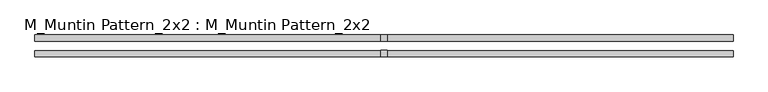
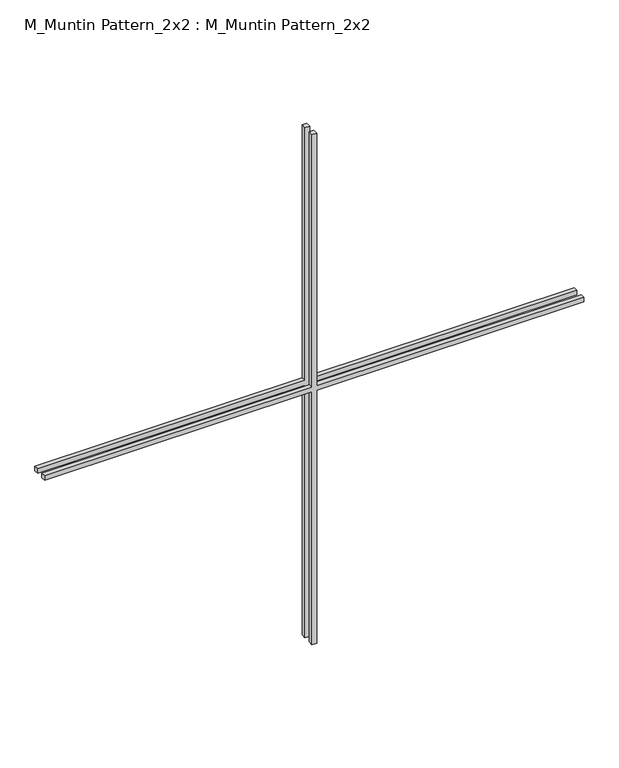
"""IFC4 building model written with IfcOpenShell, lengths in millimetres: proxy geometry, M_Muntin Pattern_2x2 : M_Muntin Pattern_2x2."""

from ifc_helpers import new_model, si_unit, frame, origin, place, context, project, spatial, polyline, outline, extrude, source, transform, mapped, element, save


def m_muntin_pattern_2x2_m_muntin_pattern_2x2_35581ed7(model_context):
    return source(origin(), model_context, "Body", "SweptSolid", [
        extrude(outline(polyline([(718.25, -6.35), (718.25, -711.9), (705.55, -711.9), (705.55, -6.35), (0.0, -6.35), (0.0, 6.35), (705.55, 6.35), (705.55, 711.9), (718.25, 711.9), (718.25, 6.35), (1423.8, 6.35), (1423.8, -6.35), (718.25, -6.35)])), frame((0.0, -22.225, 0.0), z_axis=(0.0, 1.0, 0.0), x_axis=(0.0, 0.0, 1.0)), (0.0, 0.0, 1.0), 12.7),
        extrude(outline(polyline([(718.25, -6.35), (718.25, -711.9), (705.55, -711.9), (705.55, -6.35), (0.0, -6.35), (0.0, 6.35), (705.55, 6.35), (705.55, 711.9), (718.25, 711.9), (718.25, 6.35), (1423.8, 6.35), (1423.8, -6.35), (718.25, -6.35)])), frame((0.0, 9.525, 0.0), z_axis=(0.0, 1.0, 0.0), x_axis=(0.0, 0.0, 1.0)), (0.0, 0.0, 1.0), 12.7),
    ])


if __name__ == "__main__":
    model = new_model("IFC4")
    model_context = context("Model", 3, world=origin())
    ifc_project = project(units=[si_unit("LENGTHUNIT", "METRE", prefix="MILLI")], contexts=[model_context])
    site = spatial("IfcSite", under=ifc_project)
    building = spatial("IfcBuilding", under=site)
    placement = place(None, origin())
    m_muntin_pattern_2x2_m_muntin_pattern_2x2_shape = m_muntin_pattern_2x2_m_muntin_pattern_2x2_35581ed7(model_context)
    element("IfcBuildingElementProxy", 1, Name="M_Muntin Pattern_2x2 : M_Muntin Pattern_2x2", ObjectType="M_Muntin Pattern_2x2 : M_Muntin Pattern_2x2", at=placement, inside=building, context=model_context, shape_type="MappedRepresentation", body=[
        mapped(m_muntin_pattern_2x2_m_muntin_pattern_2x2_shape, transform((0.0, 0.0, 0.0), x_axis=(1.0, 0.0, 0.0), y_axis=(0.0, 1.0, 0.0), z_axis=(0.0, 0.0, 1.0))),
    ])
    save(model, "model.ifc")

# Revit data of these elements
# Type "M_Muntin Pattern_2x2 : M_Muntin Pattern_2x2"
#   Width [instance default] = 1200 mm
#   Thickness = 12.7 mm
#   Height [instance default] = 1200 mm
#   Distance = 19.05 mm
#   Interior Material [instance default] = none
#   Exterior Material [instance default] = none
#   Default Elevation = 0
# Element 1 (IfcBuildingElementProxy, "M_Muntin Pattern_2x2 : M_Muntin Pattern_2x2")
#   Width = 1423.8 mm
#   Height = 1423.8 mm
#   Interior Material = Wood - Stained
#   Exterior Material = Clad - White
#   Materials on its faces: "Clad - White", "Wood - Stained"
# Materials
#   "Clad - White": class "Wood", colour RGB 245 245 243, transparency 0, Cost = 0
#   "Wood - Stained": class "Wood", colour RGB 173 132 96, transparency 0, Cost = 0
